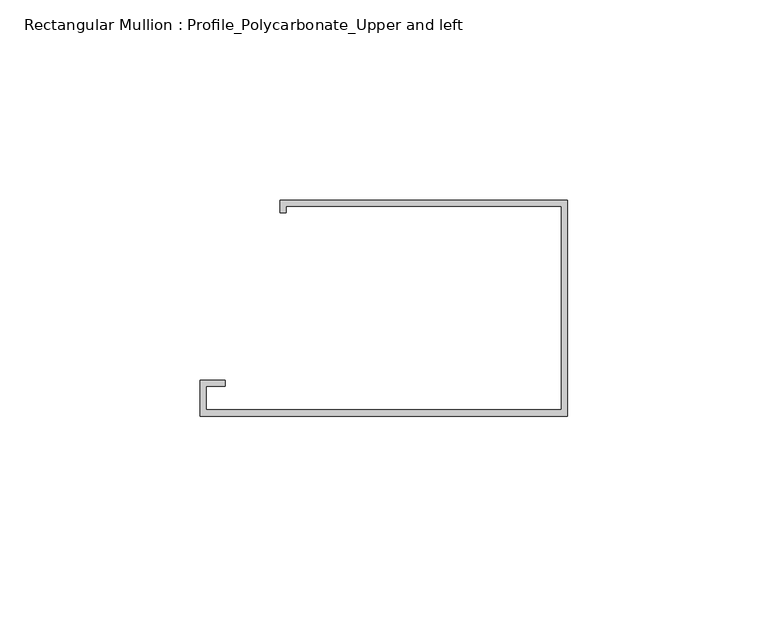
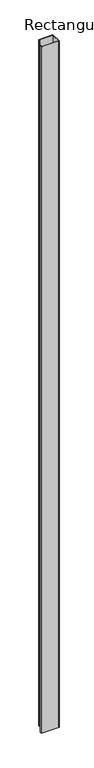
"""IFC4 building model written with IfcOpenShell, lengths in millimetres: member geometry, Rectangular Mullion : Profile_Polycarbonate_Upper and left."""

import ifcopenshell
import ifcopenshell.guid

model = None  # the IFC model being written
_history = None  # IfcOwnerHistory: only IFC2X3 demands one
_inside = {}  # id of a spatial element -> (the spatial element, [elements in it])
_under = {}  # id of a project, library or spatial element -> (it, [spatial elements below it])
_declared = {}  # id of a project -> (the project, [libraries it declares])
_typed = {}  # id of a type object -> (the type object, [elements of that type])
_made_of = {}  # id of a material, layer set ... -> (it, [elements and type objects made of it])


def new_model(schema):
    """Start an empty IFC model of exactly this schema.

    Asked for "IFC4X3", IfcOpenShell would pick the latest addendum, in which some entities
    have other attributes; the version numbers below select the first issue.
    IFC2X3 requires an IfcOwnerHistory on every rooted entity: one is made here for all.
    """
    global model, _history
    if schema == "IFC4X3":
        model = ifcopenshell.file(schema_version=(4, 3, 0, 0))
    else:
        model = ifcopenshell.file(schema=schema)
    _inside.clear()
    _under.clear()
    _declared.clear()
    _typed.clear()
    _made_of.clear()
    _history = None
    if model.schema == "IFC2X3":
        org = make("IfcOrganization", Name="unknown")
        user = make(
            "IfcPersonAndOrganization",
            ThePerson=make("IfcPerson", FamilyName="unknown"),
            TheOrganization=org,
        )
        app = make(
            "IfcApplication",
            ApplicationDeveloper=org,
            Version="unknown",
            ApplicationFullName="unknown",
            ApplicationIdentifier="unknown",
        )
        _history = make(
            "IfcOwnerHistory",
            OwningUser=user,
            OwningApplication=app,
            ChangeAction="ADDED",
            CreationDate=0,
        )
    return model


def make(cls, **values):
    """One entity of the class cls with the attributes given. An attribute that is None is left unset."""
    return model.create_entity(
        cls, **{name: value for name, value in values.items() if value is not None}
    )


def rooted(cls, **values):
    """An entity with a GlobalId (a new one), such as an element, a storey or a relation."""
    return make(cls, GlobalId=ifcopenshell.guid.new(), OwnerHistory=_history, **values)


def si_unit(unit_type, name, prefix=None):
    """IfcSIUnit, for example si_unit("LENGTHUNIT", "METRE", prefix="MILLI")."""
    return make("IfcSIUnit", UnitType=unit_type, Prefix=prefix, Name=name)


def assignment(units):
    """IfcUnitAssignment: the units of a project."""
    return None if units is None else make("IfcUnitAssignment", Units=units)


def point(xyz):
    """IfcCartesianPoint."""
    return None if xyz is None else make("IfcCartesianPoint", Coordinates=xyz)


def direction(xyz):
    """IfcDirection."""
    return None if xyz is None else make("IfcDirection", DirectionRatios=xyz)


def frame(location, z_axis=None, x_axis=None):
    """IfcAxis2Placement3D, a coordinate frame: its origin and axes. An axis left out is left unset."""
    return make(
        "IfcAxis2Placement3D",
        Location=point(location),
        Axis=direction(z_axis),
        RefDirection=direction(x_axis),
    )


def origin():
    """The frame at (0, 0, 0) with its axes left unset."""
    return frame((0.0, 0.0, 0.0))


def place(relative_to, where):
    """IfcLocalPlacement: puts the frame where relative to a parent placement (None: the world)."""
    return make(
        "IfcLocalPlacement", PlacementRelTo=relative_to, RelativePlacement=where
    )


def context(
    kind, dimensions, precision=None, world=None, true_north=None, identifier=None
):
    """IfcGeometricRepresentationContext, for example the 3D "Model" context."""
    return make(
        "IfcGeometricRepresentationContext",
        ContextIdentifier=identifier,
        ContextType=kind,
        CoordinateSpaceDimension=dimensions,
        Precision=precision,
        WorldCoordinateSystem=world,
        TrueNorth=true_north,
    )


def project(units=None, contexts=None):
    """IfcProject with its units and contexts."""
    return rooted(
        "IfcProject",
        Name="project",
        RepresentationContexts=contexts,
        UnitsInContext=assignment(units),
    )


def spatial(cls, under=None, at=None, **own):
    """A site, building, storey or space (cls), placed at a placement, below another one or the project."""
    s = rooted(cls, ObjectPlacement=at, **own)
    if under is not None:
        _under.setdefault(under.id(), (under, []))[1].append(s)
    return s


def polyline(points):
    """IfcPolyline through the points."""
    return make("IfcPolyline", Points=[point(p) for p in points])


def outline(outer, holes=None, kind="AREA"):
    """IfcArbitraryClosedProfileDef: a profile drawn as a closed curve; with holes, ...WithVoids."""
    if holes is None:
        return make("IfcArbitraryClosedProfileDef", ProfileType=kind, OuterCurve=outer)
    return make(
        "IfcArbitraryProfileDefWithVoids",
        ProfileType=kind,
        OuterCurve=outer,
        InnerCurves=holes,
    )


def extrude(swept, where, along, depth):
    """IfcExtrudedAreaSolid: the profile swept, set in the frame where, extruded along a direction by depth."""
    return make(
        "IfcExtrudedAreaSolid",
        SweptArea=swept,
        Position=where,
        ExtrudedDirection=direction(along),
        Depth=depth,
    )


def shape(context_of_items, identifier, shape_type, items):
    """IfcShapeRepresentation: the items that make up one representation, for example the "Body"."""
    return make(
        "IfcShapeRepresentation",
        ContextOfItems=context_of_items,
        RepresentationIdentifier=identifier,
        RepresentationType=shape_type,
        Items=items,
    )


def source(mapping_origin, context_of_items, identifier, shape_type, items):
    """IfcRepresentationMap: a shape defined once, which mapped items show again and again."""
    return make(
        "IfcRepresentationMap",
        MappingOrigin=mapping_origin,
        MappedRepresentation=shape(context_of_items, identifier, shape_type, items),
    )


def transform(
    local_origin,
    x_axis=None,
    y_axis=None,
    z_axis=None,
    scale=None,
    scale2=None,
    scale3=None,
    uniform=True,
):
    """IfcCartesianTransformationOperator3D, or its non-uniform kind. x_axis, y_axis, z_axis: its Axis1, 2, 3."""
    if uniform:
        return make(
            "IfcCartesianTransformationOperator3D",
            Axis1=direction(x_axis),
            Axis2=direction(y_axis),
            LocalOrigin=point(local_origin),
            Scale=scale,
            Axis3=direction(z_axis),
        )
    return make(
        "IfcCartesianTransformationOperator3DnonUniform",
        Axis1=direction(x_axis),
        Axis2=direction(y_axis),
        LocalOrigin=point(local_origin),
        Scale=scale,
        Axis3=direction(z_axis),
        Scale2=scale2,
        Scale3=scale3,
    )


def mapped(mapping_source, mapping_target):
    """IfcMappedItem: shows the shape of a source again, moved by a transform."""
    return make(
        "IfcMappedItem", MappingSource=mapping_source, MappingTarget=mapping_target
    )


def made_of(thing, what):
    """Note that an element or type object is made of a material, layer set ...; save() writes the relation."""
    if what is not None:
        _made_of.setdefault(what.id(), (what, []))[1].append(thing)
    return thing


def element(
    cls,
    number,
    at=None,
    inside=None,
    cuts=None,
    type_object=None,
    material=None,
    context=None,
    identifier="Body",
    shape_type=None,
    held_by="IfcProductDefinitionShape",
    body=None,
    shapes=None,
    **own,
):
    """One element of the class cls, such as IfcWall. Its Tag is "e" and its number.

    at: its placement. inside: the storey or other place that contains it. cuts: it is an
    opening in that element (IfcRelVoidsElement). A single representation is given by context,
    identifier, shape_type and body (its items); several are given by shapes. held_by: the class
    of the entity that holds the representations. save() writes the other relations.
    """
    e = rooted(cls, Tag="e%d" % number, ObjectPlacement=at, **own)
    if body is not None:
        shapes = [shape(context, identifier, shape_type, body)]
    if shapes is not None:
        e.Representation = make(held_by, Representations=shapes)
    if inside is not None:
        _inside.setdefault(inside.id(), (inside, []))[1].append(e)
    if cuts is not None:
        rooted(
            "IfcRelVoidsElement", RelatingBuildingElement=cuts, RelatedOpeningElement=e
        )
    if type_object is not None:
        _typed.setdefault(type_object.id(), (type_object, []))[1].append(e)
    return made_of(e, material)


def aggregate(whole, parts):
    """IfcRelAggregates: a whole, such as a stair, and the parts it consists of."""
    return rooted("IfcRelAggregates", RelatingObject=whole, RelatedObjects=parts)


def save(model, path):
    """Write the relations noted so far, then the file.

    IfcRelAggregates (storeys below a building ...), IfcRelContainedInSpatialStructure (elements
    in a storey), IfcRelDefinesByType, IfcRelAssociatesMaterial and IfcRelDeclares: one each for
    every whole, place, type object, material and project.
    """
    for whole, parts in _under.values():
        aggregate(whole, parts)
    for where, things in _inside.values():
        rooted(
            "IfcRelContainedInSpatialStructure",
            RelatedElements=things,
            RelatingStructure=where,
        )
    for kind, things in _typed.values():
        rooted("IfcRelDefinesByType", RelatedObjects=things, RelatingType=kind)
    for what, things in _made_of.values():
        rooted("IfcRelAssociatesMaterial", RelatedObjects=things, RelatingMaterial=what)
    for by, libraries in _declared.values():
        rooted("IfcRelDeclares", RelatingContext=by, RelatedDefinitions=libraries)
    model.write(path)


def rectangular_mullion_profile_polycarbonate_upper_and_left_6400ccb7(model_context):
    return source(origin(), model_context, "Body", "SweptSolid", [
        extrude(outline(polyline([(0.0, -28.984575), (-91.9988, -28.984575), (-91.9988, -19.992975), (-85.6488, -19.992975), (-85.6488, -21.580475), (-90.4113, -21.580475), (-90.4113, -27.397075), (-1.5875, -27.397075), (-1.5875, 23.428325), (-70.3961, 23.428325), (-70.3961, 21.840825), (-71.9836, 21.840825), (-71.9836, 25.015825), (0.0, 25.015825), (0.0, -28.984575)])), frame((0.0, 0.0, -3695.7), z_axis=(0.0, 0.0, 1.0), x_axis=(1.0, 0.0, 0.0)), (0.0, 0.0, 1.0), 3695.7),
    ])


if __name__ == "__main__":
    model = new_model("IFC4")
    model_context = context("Model", 3, world=origin())
    ifc_project = project(units=[si_unit("LENGTHUNIT", "METRE", prefix="MILLI")], contexts=[model_context])
    site = spatial("IfcSite", under=ifc_project)
    building = spatial("IfcBuilding", under=site)
    placement = place(None, origin())
    rectangular_mullion_profile_polycarbonate_upper_and_left_shape = rectangular_mullion_profile_polycarbonate_upper_and_left_6400ccb7(model_context)
    element("IfcMember", 1, ObjectType="Rectangular Mullion : Profile_Polycarbonate_Upper and left", at=placement, inside=building, context=model_context, shape_type="MappedRepresentation", body=[
        mapped(rectangular_mullion_profile_polycarbonate_upper_and_left_shape, transform((0.0, 0.0, 0.0), x_axis=(1.0, 0.0, 0.0), y_axis=(0.0, 1.0, 0.0), z_axis=(0.0, 0.0, 1.0))),
    ])
    save(model, "model.ifc")

# Revit data of these elements
# Type "Rectangular Mullion : Profile_Polycarbonate_Upper and left"
#   built-in parameter 1007322 = 0.177167 (stored number, unit not read)
#   built-in parameter 1007321 = 0.00520833 (stored number, unit not read)
#   built-in parameter 1007320 = 0 (stored number, unit not read)
